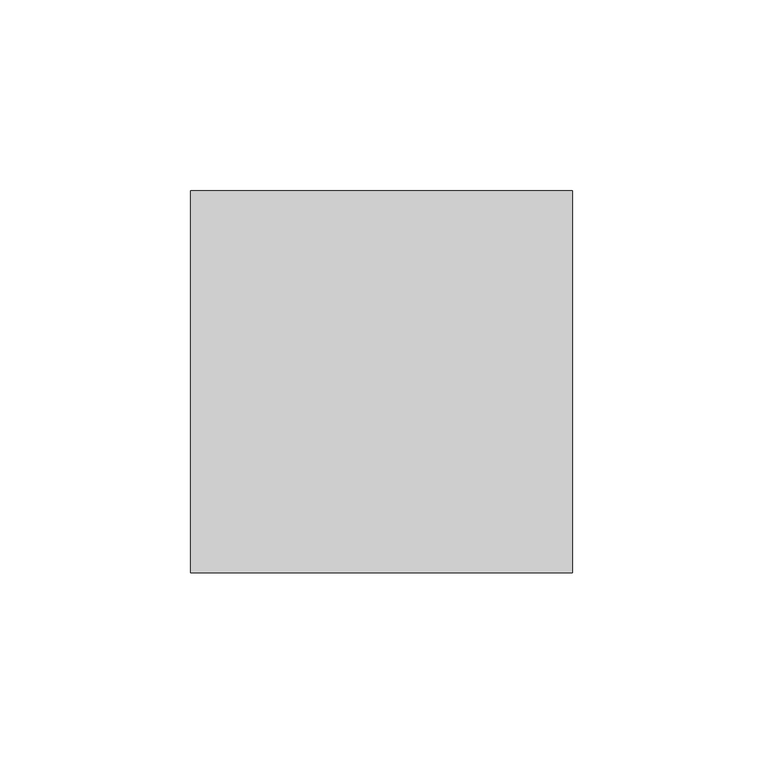
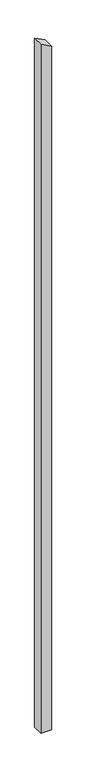
"""IFC4 building model written with IfcOpenShell, lengths in millimetres: column geometry, Holzstütze 159106 : Holzstütze 159106."""

import ifcopenshell
import ifcopenshell.guid

model = None  # the IFC model being written
_history = None  # IfcOwnerHistory: only IFC2X3 demands one
_inside = {}  # id of a spatial element -> (the spatial element, [elements in it])
_under = {}  # id of a project, library or spatial element -> (it, [spatial elements below it])
_declared = {}  # id of a project -> (the project, [libraries it declares])
_typed = {}  # id of a type object -> (the type object, [elements of that type])
_made_of = {}  # id of a material, layer set ... -> (it, [elements and type objects made of it])


def new_model(schema):
    """Start an empty IFC model of exactly this schema.

    Asked for "IFC4X3", IfcOpenShell would pick the latest addendum, in which some entities
    have other attributes; the version numbers below select the first issue.
    IFC2X3 requires an IfcOwnerHistory on every rooted entity: one is made here for all.
    """
    global model, _history
    if schema == "IFC4X3":
        model = ifcopenshell.file(schema_version=(4, 3, 0, 0))
    else:
        model = ifcopenshell.file(schema=schema)
    _inside.clear()
    _under.clear()
    _declared.clear()
    _typed.clear()
    _made_of.clear()
    _history = None
    if model.schema == "IFC2X3":
        org = make("IfcOrganization", Name="unknown")
        user = make(
            "IfcPersonAndOrganization",
            ThePerson=make("IfcPerson", FamilyName="unknown"),
            TheOrganization=org,
        )
        app = make(
            "IfcApplication",
            ApplicationDeveloper=org,
            Version="unknown",
            ApplicationFullName="unknown",
            ApplicationIdentifier="unknown",
        )
        _history = make(
            "IfcOwnerHistory",
            OwningUser=user,
            OwningApplication=app,
            ChangeAction="ADDED",
            CreationDate=0,
        )
    return model


def make(cls, **values):
    """One entity of the class cls with the attributes given. An attribute that is None is left unset."""
    return model.create_entity(
        cls, **{name: value for name, value in values.items() if value is not None}
    )


def rooted(cls, **values):
    """An entity with a GlobalId (a new one), such as an element, a storey or a relation."""
    return make(cls, GlobalId=ifcopenshell.guid.new(), OwnerHistory=_history, **values)


def si_unit(unit_type, name, prefix=None):
    """IfcSIUnit, for example si_unit("LENGTHUNIT", "METRE", prefix="MILLI")."""
    return make("IfcSIUnit", UnitType=unit_type, Prefix=prefix, Name=name)


def assignment(units):
    """IfcUnitAssignment: the units of a project."""
    return None if units is None else make("IfcUnitAssignment", Units=units)


def point(xyz):
    """IfcCartesianPoint."""
    return None if xyz is None else make("IfcCartesianPoint", Coordinates=xyz)


def direction(xyz):
    """IfcDirection."""
    return None if xyz is None else make("IfcDirection", DirectionRatios=xyz)


def frame(location, z_axis=None, x_axis=None):
    """IfcAxis2Placement3D, a coordinate frame: its origin and axes. An axis left out is left unset."""
    return make(
        "IfcAxis2Placement3D",
        Location=point(location),
        Axis=direction(z_axis),
        RefDirection=direction(x_axis),
    )


def origin():
    """The frame at (0, 0, 0) with its axes left unset."""
    return frame((0.0, 0.0, 0.0))


def place(relative_to, where):
    """IfcLocalPlacement: puts the frame where relative to a parent placement (None: the world)."""
    return make(
        "IfcLocalPlacement", PlacementRelTo=relative_to, RelativePlacement=where
    )


def context(
    kind, dimensions, precision=None, world=None, true_north=None, identifier=None
):
    """IfcGeometricRepresentationContext, for example the 3D "Model" context."""
    return make(
        "IfcGeometricRepresentationContext",
        ContextIdentifier=identifier,
        ContextType=kind,
        CoordinateSpaceDimension=dimensions,
        Precision=precision,
        WorldCoordinateSystem=world,
        TrueNorth=true_north,
    )


def project(units=None, contexts=None):
    """IfcProject with its units and contexts."""
    return rooted(
        "IfcProject",
        Name="project",
        RepresentationContexts=contexts,
        UnitsInContext=assignment(units),
    )


def spatial(cls, under=None, at=None, **own):
    """A site, building, storey or space (cls), placed at a placement, below another one or the project."""
    s = rooted(cls, ObjectPlacement=at, **own)
    if under is not None:
        _under.setdefault(under.id(), (under, []))[1].append(s)
    return s


def polyline(points):
    """IfcPolyline through the points."""
    return make("IfcPolyline", Points=[point(p) for p in points])


def outline(outer, holes=None, kind="AREA"):
    """IfcArbitraryClosedProfileDef: a profile drawn as a closed curve; with holes, ...WithVoids."""
    if holes is None:
        return make("IfcArbitraryClosedProfileDef", ProfileType=kind, OuterCurve=outer)
    return make(
        "IfcArbitraryProfileDefWithVoids",
        ProfileType=kind,
        OuterCurve=outer,
        InnerCurves=holes,
    )


def extrude(swept, where, along, depth):
    """IfcExtrudedAreaSolid: the profile swept, set in the frame where, extruded along a direction by depth."""
    return make(
        "IfcExtrudedAreaSolid",
        SweptArea=swept,
        Position=where,
        ExtrudedDirection=direction(along),
        Depth=depth,
    )


def shape(context_of_items, identifier, shape_type, items):
    """IfcShapeRepresentation: the items that make up one representation, for example the "Body"."""
    return make(
        "IfcShapeRepresentation",
        ContextOfItems=context_of_items,
        RepresentationIdentifier=identifier,
        RepresentationType=shape_type,
        Items=items,
    )


def source(mapping_origin, context_of_items, identifier, shape_type, items):
    """IfcRepresentationMap: a shape defined once, which mapped items show again and again."""
    return make(
        "IfcRepresentationMap",
        MappingOrigin=mapping_origin,
        MappedRepresentation=shape(context_of_items, identifier, shape_type, items),
    )


def transform(
    local_origin,
    x_axis=None,
    y_axis=None,
    z_axis=None,
    scale=None,
    scale2=None,
    scale3=None,
    uniform=True,
):
    """IfcCartesianTransformationOperator3D, or its non-uniform kind. x_axis, y_axis, z_axis: its Axis1, 2, 3."""
    if uniform:
        return make(
            "IfcCartesianTransformationOperator3D",
            Axis1=direction(x_axis),
            Axis2=direction(y_axis),
            LocalOrigin=point(local_origin),
            Scale=scale,
            Axis3=direction(z_axis),
        )
    return make(
        "IfcCartesianTransformationOperator3DnonUniform",
        Axis1=direction(x_axis),
        Axis2=direction(y_axis),
        LocalOrigin=point(local_origin),
        Scale=scale,
        Axis3=direction(z_axis),
        Scale2=scale2,
        Scale3=scale3,
    )


def mapped(mapping_source, mapping_target):
    """IfcMappedItem: shows the shape of a source again, moved by a transform."""
    return make(
        "IfcMappedItem", MappingSource=mapping_source, MappingTarget=mapping_target
    )


def made_of(thing, what):
    """Note that an element or type object is made of a material, layer set ...; save() writes the relation."""
    if what is not None:
        _made_of.setdefault(what.id(), (what, []))[1].append(thing)
    return thing


def element(
    cls,
    number,
    at=None,
    inside=None,
    cuts=None,
    type_object=None,
    material=None,
    context=None,
    identifier="Body",
    shape_type=None,
    held_by="IfcProductDefinitionShape",
    body=None,
    shapes=None,
    **own,
):
    """One element of the class cls, such as IfcWall. Its Tag is "e" and its number.

    at: its placement. inside: the storey or other place that contains it. cuts: it is an
    opening in that element (IfcRelVoidsElement). A single representation is given by context,
    identifier, shape_type and body (its items); several are given by shapes. held_by: the class
    of the entity that holds the representations. save() writes the other relations.
    """
    e = rooted(cls, Tag="e%d" % number, ObjectPlacement=at, **own)
    if body is not None:
        shapes = [shape(context, identifier, shape_type, body)]
    if shapes is not None:
        e.Representation = make(held_by, Representations=shapes)
    if inside is not None:
        _inside.setdefault(inside.id(), (inside, []))[1].append(e)
    if cuts is not None:
        rooted(
            "IfcRelVoidsElement", RelatingBuildingElement=cuts, RelatedOpeningElement=e
        )
    if type_object is not None:
        _typed.setdefault(type_object.id(), (type_object, []))[1].append(e)
    return made_of(e, material)


def aggregate(whole, parts):
    """IfcRelAggregates: a whole, such as a stair, and the parts it consists of."""
    return rooted("IfcRelAggregates", RelatingObject=whole, RelatedObjects=parts)


def save(model, path):
    """Write the relations noted so far, then the file.

    IfcRelAggregates (storeys below a building ...), IfcRelContainedInSpatialStructure (elements
    in a storey), IfcRelDefinesByType, IfcRelAssociatesMaterial and IfcRelDeclares: one each for
    every whole, place, type object, material and project.
    """
    for whole, parts in _under.values():
        aggregate(whole, parts)
    for where, things in _inside.values():
        rooted(
            "IfcRelContainedInSpatialStructure",
            RelatedElements=things,
            RelatingStructure=where,
        )
    for kind, things in _typed.values():
        rooted("IfcRelDefinesByType", RelatedObjects=things, RelatingType=kind)
    for what, things in _made_of.values():
        rooted("IfcRelAssociatesMaterial", RelatedObjects=things, RelatingMaterial=what)
    for by, libraries in _declared.values():
        rooted("IfcRelDeclares", RelatingContext=by, RelatedDefinitions=libraries)
    model.write(path)


def column_a4466fb5(model_context):
    return source(origin(), model_context, "Body", "SweptSolid", [
        extrude(outline(polyline([(-500.0, 174197.7593015), (-500.0, 174297.7593015), (6345.7118258, 174297.7593015), (6396.6643707, 174197.7593015), (-500.0, 174197.7593015)])), frame((0.0, 31941.5369795, 0.0), z_axis=(0.0, 1.0, 0.0), x_axis=(0.0, 0.0, 1.0)), (0.0, 0.0, 1.0), 100.0),
    ])


if __name__ == "__main__":
    model = new_model("IFC4")
    model_context = context("Model", 3, world=origin())
    ifc_project = project(units=[si_unit("LENGTHUNIT", "METRE", prefix="MILLI")], contexts=[model_context])
    site = spatial("IfcSite", under=ifc_project)
    building = spatial("IfcBuilding", under=site)
    placement = place(None, origin())
    column_shape = column_a4466fb5(model_context)
    element("IfcColumn", 1, ObjectType="Holzstütze 159106 : Holzstütze 159106", at=placement, inside=building, context=model_context, shape_type="MappedRepresentation", body=[
        mapped(column_shape, transform((0.0, 0.0, 0.0), x_axis=(1.0, 0.0, 0.0), y_axis=(0.0, 1.0, 0.0), z_axis=(0.0, 0.0, 1.0))),
    ])
    save(model, "model.ifc")

# Revit data of these elements
# Type "Holzstütze 159106 : Holzstütze 159106"
#   Abrechnungsart = "m"
#   Allright_Bauteil_ID = "0152St 0000143487"
#   Bezeichnung = "Holzstütze"
#   Codetext = "ST-HOLZ\\"
#   Gewerk = "Zimmer- und Holzbauarbeiten"
#   Material = "Holz"
#   Objektname = "Stütze"
#   NameOverride = "Holzstütze"
#   Reference = "Holzstütze"
#   Status = "NEW"
#   ThermalTransmittance = 0.0000 BTU/(h·ft²·°F)
#   Roll = 0.00°
#   Slope = 0.00°
#   2D Interaktion = yes
#   IsExternal = yes
#   LoadBearing = yes
# Element 1 (IfcColumn, "Holzstütze 159106 : Holzstütze 159106")
#   Materials on its faces: "holzschalung"
# Materials
#   "holzschalung": class "Unassigned", colour RGB 128 128 128, transparency 0
